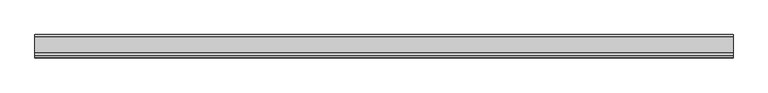
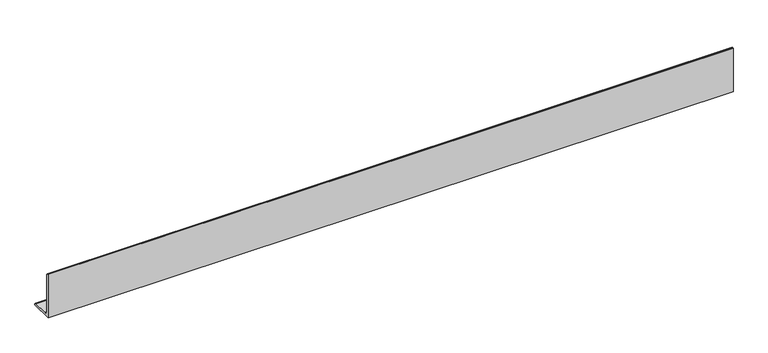
"""IFC4 building model written with IfcOpenShell, lengths in millimetres: beam geometry, NLRS_28_SF_LIB_stalen ligger hoekprofiel ongelijkzijdig-AV-MMBS-SRP_gen_rsf : stalen ligger ongelijzijdig hoekprofiel LUEQ_gen__200x100x10."""

from ifc_helpers import new_model, si_unit, point, frame, frame_2d, origin, place, context, project, spatial, polyline, circle_curve, trimmed, segment, composite_curve, outline, extrude, source, transform, mapped, element, save


def beam_d9217694(model_context):
    return source(origin(), model_context, "Body", "SweptSolid", [
        extrude(outline(composite_curve([segment(polyline([(-20.13, -69.3), (-20.13, 130.7), (-17.63, 130.7)]), True, "CONTINUOUS"), segment(trimmed(circle_curve(frame_2d((-17.63, 123.2)), 7.5), [point((-17.63, 130.7))], [point((-10.13, 123.2))], False, "CARTESIAN"), True, "CONTINUOUS"), segment(polyline([(-10.13, 123.2), (-10.13, -44.3)]), True, "CONTINUOUS"), segment(trimmed(circle_curve(frame_2d((4.87, -44.3)), 15.0), [point((-10.13, -44.3))], [point((4.87, -59.3))], True, "CARTESIAN"), True, "CONTINUOUS"), segment(polyline([(4.87, -59.3), (72.37, -59.3)]), True, "CONTINUOUS"), segment(trimmed(circle_curve(frame_2d((72.37, -66.8)), 7.5), [point((72.37, -59.3))], [point((79.87, -66.8))], False, "CARTESIAN"), True, "CONTINUOUS"), segment(polyline([(79.87, -66.8), (79.87, -69.3), (-20.13, -69.3)]), True, "CONTINUOUS")], self_intersect=False)), frame((-1482.2999994, 0.0, 0.0), z_axis=(1.0, 0.0, 0.0), x_axis=(0.0, 1.0, 0.0)), (0.0, 0.0, 1.0), 2977.2999994),
    ])


if __name__ == "__main__":
    model = new_model("IFC4")
    model_context = context("Model", 3, world=origin())
    ifc_project = project(units=[si_unit("LENGTHUNIT", "METRE", prefix="MILLI")], contexts=[model_context])
    site = spatial("IfcSite", under=ifc_project)
    building = spatial("IfcBuilding", under=site)
    placement = place(None, origin())
    beam_shape = beam_d9217694(model_context)
    element("IfcBeam", 1, ObjectType="NLRS_28_SF_LIB_stalen ligger hoekprofiel ongelijkzijdig-AV-MMBS-SRP_gen_rsf : stalen ligger ongelijzijdig hoekprofiel LUEQ_gen__200x100x10", at=placement, inside=building, context=model_context, shape_type="MappedRepresentation", body=[
        mapped(beam_shape, transform((0.0, 0.0, 0.0), x_axis=(1.0, 0.0, 0.0), y_axis=(0.0, 1.0, 0.0), z_axis=(0.0, 0.0, 1.0))),
    ])
    save(model, "model.ifc")

# Revit data of these elements
# Type "NLRS_28_SF_LIB_stalen ligger hoekprofiel ongelijkzijdig-AV-MMBS-SRP_gen_rsf : stalen ligger ongelijzijdig hoekprofiel LUEQ_gen__200x100x10"
#   Type IfcGUID = "0dxhH9VHH5jh7XQ0uLfXuR"
#   IfcExportAs = "IfcBeamType"
#   Type Comments = "L200x100x10"
#   Model = " "
#   Manufacturer = " "
#   Fire Rating = " "
#   Description = "stalen ligger L200x100x10"
#   Assembly Code = "28.11"
#   vz = 130.7 mm
#   vy = 79.87 mm
#   tw = 10 mm
#   tf = 10 mm
#   ri = 7.5 mm
#   ra = 15 mm
#   d = 200 mm
#   bf = 100 mm
#   NLRS_C_lengte [instance default] = 1524 mm
#   Length [instance default] = 1524 mm
#   Structural Material = NLRS_h2_staal_gen_rsf
#   Keynote = ""
# Element 1 (IfcBeam, "NLRS_28_SF_LIB_stalen ligger hoekprofiel ongelijkzijdig-AV-MMBS-SRP_gen_rsf : stalen ligger ongelijzijdig hoekprofiel LUEQ_gen__200x100x10")
#   NLRS_C_lengte = 2990 mm
#   Materials on its faces: "NLRS_h2_staal_gen_rsf"
# Materials
#   "NLRS_h2_staal_gen_rsf": class "H - Metaal", colour RGB 189 187 185, transparency 0, Keynote = "h2", Manufacturer = "Revit Standards Foundation", URL = "www.revitstandards.org", Description = "staal", Cost = 0
